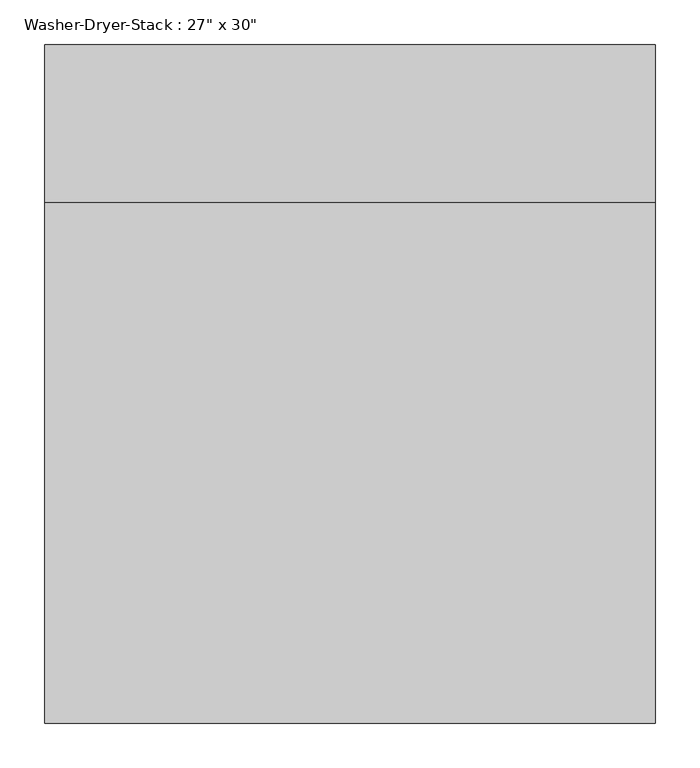
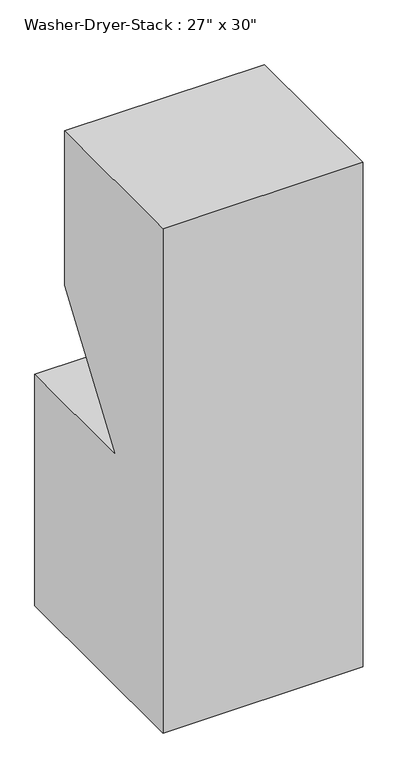
"""IFC4 building model written with IfcOpenShell, lengths in millimetres: proxy geometry."""

from ifc_helpers import new_model, si_unit, frame, origin, place, context, project, spatial, polyline, outline, extrude, source, transform, mapped, element, save


def proxy_5c28bc07(model_context):
    return source(origin(), model_context, "Body", "SweptSolid", [
        extrude(outline(polyline([(381.0, 0.0), (-381.0, 0.0), (-381.0, 1828.8), (203.2, 1828.8), (203.2, 1270.0), (-99.149615, 838.2), (381.0, 838.2), (381.0, 0.0)])), frame((-342.9, 0.0, 0.0), z_axis=(1.0, 0.0, 0.0), x_axis=(0.0, 1.0, 0.0)), (0.0, 0.0, 1.0), 685.8),
    ])


if __name__ == "__main__":
    model = new_model("IFC4")
    model_context = context("Model", 3, world=origin())
    ifc_project = project(units=[si_unit("LENGTHUNIT", "METRE", prefix="MILLI")], contexts=[model_context])
    site = spatial("IfcSite", under=ifc_project)
    building = spatial("IfcBuilding", under=site)
    placement = place(None, origin())
    proxy_shape = proxy_5c28bc07(model_context)
    element("IfcBuildingElementProxy", 1, Name="Washer-Dryer-Stack : 27\" x 30\"", ObjectType="Washer-Dryer-Stack : 27\" x 30\"", at=placement, inside=building, context=model_context, shape_type="MappedRepresentation", body=[
        mapped(proxy_shape, transform((0.0, 0.0, 0.0), x_axis=(1.0, 0.0, 0.0), y_axis=(0.0, 1.0, 0.0), z_axis=(0.0, 0.0, 1.0))),
    ])
    save(model, "model.ifc")

# Revit data of these elements
# Type "Washer-Dryer-Stack : 27\" x 30\""
#   Assembly Code = "E1090400"
#   Lower Depth = 2' - 6"
#   Upper Depth = 1' - 11"
#   Width = 2' - 3"
#   Material = STACKABLE WASHER/DRYER
# Element 1 (IfcBuildingElementProxy, "Washer-Dryer-Stack : 27\" x 30\"")
#   Materials on its faces: "STACKABLE WASHER/DRYER"
# Materials
#   "STACKABLE WASHER/DRYER": class "Metal", colour RGB 247 247 239, transparency 0, Cost = 0
